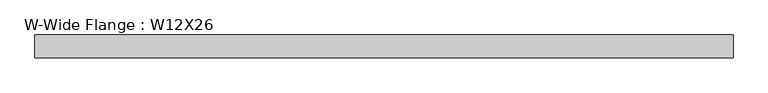
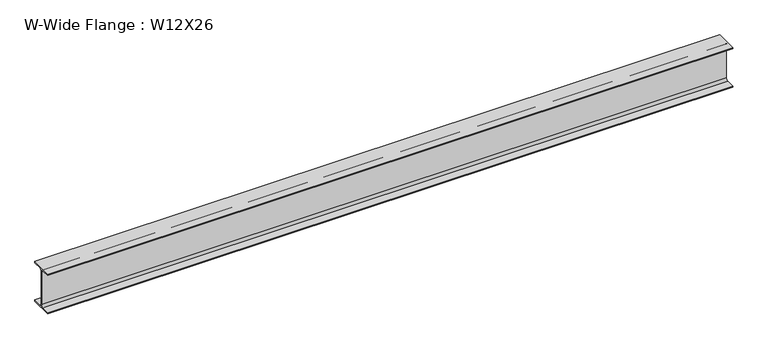
"""IFC4 building model written with IfcOpenShell, lengths in millimetres: beam geometry, W-Wide Flange : W12X26."""

from ifc_helpers import new_model, si_unit, point, frame, frame_2d, origin, place, context, project, spatial, polyline, circle_curve, trimmed, segment, composite_curve, outline, extrude, source, transform, mapped, element, save


def w_wide_flange_w12x26_dc644cb4(model_context):
    return source(origin(), model_context, "Body", "SweptSolid", [
        extrude(outline(composite_curve([segment(polyline([(82.4011719, -145.5539063), (82.4011719, -155.178125), (-82.4011719, -155.178125), (-82.4011719, -145.5539063), (-20.2902344, -145.5539063)]), True, "CONTINUOUS"), segment(trimmed(circle_curve(frame_2d((-20.2902344, -128.190625)), 17.3632812), [point((-20.2902344, -145.5539063))], [point((-2.9269531, -128.190625))], True, "CARTESIAN"), True, "CONTINUOUS"), segment(polyline([(-2.9269531, -128.190625), (-2.9269531, 128.190625)]), True, "CONTINUOUS"), segment(trimmed(circle_curve(frame_2d((-20.2902344, 128.190625)), 17.3632812), [point((-2.9269531, 128.190625))], [point((-20.2902344, 145.5539062))], True, "CARTESIAN"), True, "CONTINUOUS"), segment(polyline([(-20.2902344, 145.5539062), (-82.4011719, 145.5539062), (-82.4011719, 155.178125), (82.4011719, 155.178125), (82.4011719, 145.5539062), (20.2902344, 145.5539062)]), True, "CONTINUOUS"), segment(trimmed(circle_curve(frame_2d((20.2902344, 128.190625)), 17.3632812), [point((20.2902344, 145.5539062))], [point((2.9269531, 128.190625))], True, "CARTESIAN"), True, "CONTINUOUS"), segment(polyline([(2.9269531, 128.190625), (2.9269531, -128.190625)]), True, "CONTINUOUS"), segment(trimmed(circle_curve(frame_2d((20.2902344, -128.190625)), 17.3632812), [point((2.9269531, -128.190625))], [point((20.2902344, -145.5539063))], True, "CARTESIAN"), True, "CONTINUOUS"), segment(polyline([(20.2902344, -145.5539063), (82.4011719, -145.5539063)]), True, "CONTINUOUS")], self_intersect=False)), frame((-3644.9000006, 0.0, 0.0), z_axis=(1.0, 0.0, 0.0), x_axis=(0.0, 1.0, 0.0)), (0.0, 0.0, 1.0), 5060.9500006),
    ])


if __name__ == "__main__":
    model = new_model("IFC4")
    model_context = context("Model", 3, world=origin())
    ifc_project = project(units=[si_unit("LENGTHUNIT", "METRE", prefix="MILLI")], contexts=[model_context])
    site = spatial("IfcSite", under=ifc_project)
    building = spatial("IfcBuilding", under=site)
    placement = place(None, origin())
    w_wide_flange_w12x26_shape = w_wide_flange_w12x26_dc644cb4(model_context)
    element("IfcBeam", 1, ObjectType="W-Wide Flange : W12X26", at=placement, inside=building, context=model_context, shape_type="MappedRepresentation", body=[
        mapped(w_wide_flange_w12x26_shape, transform((0.0, 0.0, 0.0), x_axis=(1.0, 0.0, 0.0), y_axis=(0.0, 1.0, 0.0), z_axis=(0.0, 0.0, 1.0))),
    ])
    save(model, "model.ifc")

# Revit data of these elements
# Type "W-Wide Flange : W12X26"
#   Assembly Code = "B10"
#   W = 26
#   Length [instance default] = 5' - 0"
#   bf = 0' - 6 125/256"
#   d = 1' - 0 7/32"
#   k = 0' - 1 1/16"
#   k2 = 0' - 0 175/256"
#   tf = 0' - 0 97/256"
#   tw = 0' - 0 59/256"
#   A = 0.053125 SF
#   Structural Material [instance default] = none
# Element 1 (IfcBeam, "W-Wide Flange : W12X26")
#   Structural Material = PAINTED STEEL
#   Materials on its faces: "PAINTED STEEL"
# Materials
#   "PAINTED STEEL": class "Generic", colour RGB 120 120 120, transparency 0, Cost = 0
